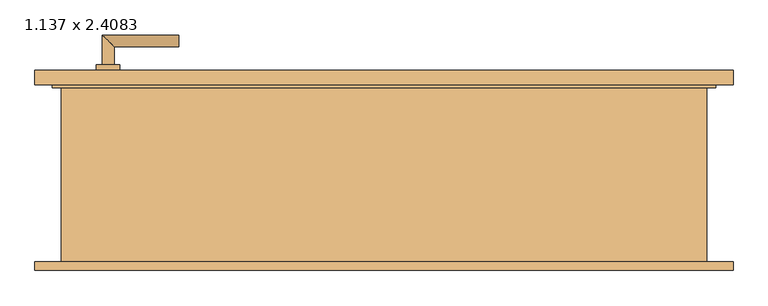
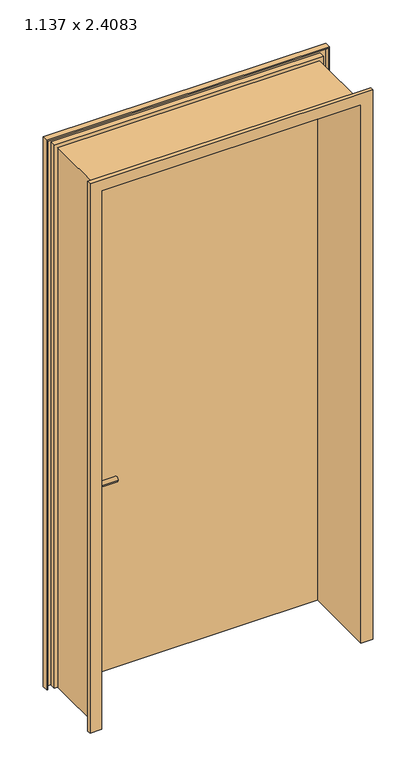
"""IFC4 building model written with IfcOpenShell, lengths in millimetres: door geometry, Drehflügel 1-flg - Stahlzarge : 1.137 x 2.4083."""

import ifcopenshell
import ifcopenshell.guid

model = None  # the IFC model being written
_history = None  # IfcOwnerHistory: only IFC2X3 demands one
_inside = {}  # id of a spatial element -> (the spatial element, [elements in it])
_under = {}  # id of a project, library or spatial element -> (it, [spatial elements below it])
_declared = {}  # id of a project -> (the project, [libraries it declares])
_typed = {}  # id of a type object -> (the type object, [elements of that type])
_made_of = {}  # id of a material, layer set ... -> (it, [elements and type objects made of it])


def new_model(schema):
    """Start an empty IFC model of exactly this schema.

    Asked for "IFC4X3", IfcOpenShell would pick the latest addendum, in which some entities
    have other attributes; the version numbers below select the first issue.
    IFC2X3 requires an IfcOwnerHistory on every rooted entity: one is made here for all.
    """
    global model, _history
    if schema == "IFC4X3":
        model = ifcopenshell.file(schema_version=(4, 3, 0, 0))
    else:
        model = ifcopenshell.file(schema=schema)
    _inside.clear()
    _under.clear()
    _declared.clear()
    _typed.clear()
    _made_of.clear()
    _history = None
    if model.schema == "IFC2X3":
        org = make("IfcOrganization", Name="unknown")
        user = make(
            "IfcPersonAndOrganization",
            ThePerson=make("IfcPerson", FamilyName="unknown"),
            TheOrganization=org,
        )
        app = make(
            "IfcApplication",
            ApplicationDeveloper=org,
            Version="unknown",
            ApplicationFullName="unknown",
            ApplicationIdentifier="unknown",
        )
        _history = make(
            "IfcOwnerHistory",
            OwningUser=user,
            OwningApplication=app,
            ChangeAction="ADDED",
            CreationDate=0,
        )
    return model


def make(cls, **values):
    """One entity of the class cls with the attributes given. An attribute that is None is left unset."""
    return model.create_entity(
        cls, **{name: value for name, value in values.items() if value is not None}
    )


def rooted(cls, **values):
    """An entity with a GlobalId (a new one), such as an element, a storey or a relation."""
    return make(cls, GlobalId=ifcopenshell.guid.new(), OwnerHistory=_history, **values)


def si_unit(unit_type, name, prefix=None):
    """IfcSIUnit, for example si_unit("LENGTHUNIT", "METRE", prefix="MILLI")."""
    return make("IfcSIUnit", UnitType=unit_type, Prefix=prefix, Name=name)


def assignment(units):
    """IfcUnitAssignment: the units of a project."""
    return None if units is None else make("IfcUnitAssignment", Units=units)


def point(xyz):
    """IfcCartesianPoint."""
    return None if xyz is None else make("IfcCartesianPoint", Coordinates=xyz)


def direction(xyz):
    """IfcDirection."""
    return None if xyz is None else make("IfcDirection", DirectionRatios=xyz)


def frame(location, z_axis=None, x_axis=None):
    """IfcAxis2Placement3D, a coordinate frame: its origin and axes. An axis left out is left unset."""
    return make(
        "IfcAxis2Placement3D",
        Location=point(location),
        Axis=direction(z_axis),
        RefDirection=direction(x_axis),
    )


def frame_2d(location, x_axis=None):
    """IfcAxis2Placement2D, a coordinate frame in the plane: its origin and x axis."""
    return make(
        "IfcAxis2Placement2D", Location=point(location), RefDirection=direction(x_axis)
    )


def origin():
    """The frame at (0, 0, 0) with its axes left unset."""
    return frame((0.0, 0.0, 0.0))


def place(relative_to, where):
    """IfcLocalPlacement: puts the frame where relative to a parent placement (None: the world)."""
    return make(
        "IfcLocalPlacement", PlacementRelTo=relative_to, RelativePlacement=where
    )


def context(
    kind, dimensions, precision=None, world=None, true_north=None, identifier=None
):
    """IfcGeometricRepresentationContext, for example the 3D "Model" context."""
    return make(
        "IfcGeometricRepresentationContext",
        ContextIdentifier=identifier,
        ContextType=kind,
        CoordinateSpaceDimension=dimensions,
        Precision=precision,
        WorldCoordinateSystem=world,
        TrueNorth=true_north,
    )


def project(units=None, contexts=None):
    """IfcProject with its units and contexts."""
    return rooted(
        "IfcProject",
        Name="project",
        RepresentationContexts=contexts,
        UnitsInContext=assignment(units),
    )


def spatial(cls, under=None, at=None, **own):
    """A site, building, storey or space (cls), placed at a placement, below another one or the project."""
    s = rooted(cls, ObjectPlacement=at, **own)
    if under is not None:
        _under.setdefault(under.id(), (under, []))[1].append(s)
    return s


def polyline(points):
    """IfcPolyline through the points."""
    return make("IfcPolyline", Points=[point(p) for p in points])


def circle_curve(where, radius):
    """IfcCircle in the frame where."""
    return make("IfcCircle", Position=where, Radius=radius)


def ellipse_curve(where, semi_axis1, semi_axis2):
    """IfcEllipse in the frame where."""
    return make(
        "IfcEllipse", Position=where, SemiAxis1=semi_axis1, SemiAxis2=semi_axis2
    )


def trimmed(basis, trim1, trim2, sense, master):
    """IfcTrimmedCurve: the piece of a basis curve between two trims."""
    return make(
        "IfcTrimmedCurve",
        BasisCurve=basis,
        Trim1=trim1,
        Trim2=trim2,
        SenseAgreement=sense,
        MasterRepresentation=master,
    )


def segment(curve, same_sense, transition):
    """IfcCompositeCurveSegment."""
    return make(
        "IfcCompositeCurveSegment",
        Transition=transition,
        SameSense=same_sense,
        ParentCurve=curve,
    )


def composite_curve(segments, self_intersect=None):
    """IfcCompositeCurve: segments joined end to end."""
    return make("IfcCompositeCurve", Segments=segments, SelfIntersect=self_intersect)


def outline(outer, holes=None, kind="AREA"):
    """IfcArbitraryClosedProfileDef: a profile drawn as a closed curve; with holes, ...WithVoids."""
    if holes is None:
        return make("IfcArbitraryClosedProfileDef", ProfileType=kind, OuterCurve=outer)
    return make(
        "IfcArbitraryProfileDefWithVoids",
        ProfileType=kind,
        OuterCurve=outer,
        InnerCurves=holes,
    )


def extrude(swept, where, along, depth):
    """IfcExtrudedAreaSolid: the profile swept, set in the frame where, extruded along a direction by depth."""
    return make(
        "IfcExtrudedAreaSolid",
        SweptArea=swept,
        Position=where,
        ExtrudedDirection=direction(along),
        Depth=depth,
    )


def faces_of(points, faces, orient=None, outer=None):
    """IfcFace entities. A face is a list of loops; a loop is a list of indices into points, from 0.

    orient and outer hold one flag for each loop. By default every Orientation is true, the
    first loop of a face is its IfcFaceOuterBound and the others are IfcFaceBound.
    """
    made = []
    for i, loops in enumerate(faces):
        bounds = []
        for j, loop in enumerate(loops):
            is_outer = j == 0 if outer is None else outer[i][j]
            bounds.append(
                make(
                    "IfcFaceOuterBound" if is_outer else "IfcFaceBound",
                    Bound=make("IfcPolyLoop", Polygon=[points[k] for k in loop]),
                    Orientation=True if orient is None else orient[i][j],
                )
            )
        made.append(make("IfcFace", Bounds=bounds))
    return made


def faceted_brep(points, faces, orient=None, outer=None, voids=None):
    """IfcFacetedBrep: a solid bounded by flat faces; with voids (closed shells), ...WithVoids."""
    shared = [point(p) for p in points]
    hull = make("IfcClosedShell", CfsFaces=faces_of(shared, faces, orient, outer))
    if voids is None:
        return make("IfcFacetedBrep", Outer=hull)
    return make(
        "IfcFacetedBrepWithVoids",
        Outer=hull,
        Voids=[
            make(cls, CfsFaces=faces_of(shared, fs, o, b)) for cls, fs, o, b in voids
        ],
    )


def shape(context_of_items, identifier, shape_type, items):
    """IfcShapeRepresentation: the items that make up one representation, for example the "Body"."""
    return make(
        "IfcShapeRepresentation",
        ContextOfItems=context_of_items,
        RepresentationIdentifier=identifier,
        RepresentationType=shape_type,
        Items=items,
    )


def source(mapping_origin, context_of_items, identifier, shape_type, items):
    """IfcRepresentationMap: a shape defined once, which mapped items show again and again."""
    return make(
        "IfcRepresentationMap",
        MappingOrigin=mapping_origin,
        MappedRepresentation=shape(context_of_items, identifier, shape_type, items),
    )


def transform(
    local_origin,
    x_axis=None,
    y_axis=None,
    z_axis=None,
    scale=None,
    scale2=None,
    scale3=None,
    uniform=True,
):
    """IfcCartesianTransformationOperator3D, or its non-uniform kind. x_axis, y_axis, z_axis: its Axis1, 2, 3."""
    if uniform:
        return make(
            "IfcCartesianTransformationOperator3D",
            Axis1=direction(x_axis),
            Axis2=direction(y_axis),
            LocalOrigin=point(local_origin),
            Scale=scale,
            Axis3=direction(z_axis),
        )
    return make(
        "IfcCartesianTransformationOperator3DnonUniform",
        Axis1=direction(x_axis),
        Axis2=direction(y_axis),
        LocalOrigin=point(local_origin),
        Scale=scale,
        Axis3=direction(z_axis),
        Scale2=scale2,
        Scale3=scale3,
    )


def mapped(mapping_source, mapping_target):
    """IfcMappedItem: shows the shape of a source again, moved by a transform."""
    return make(
        "IfcMappedItem", MappingSource=mapping_source, MappingTarget=mapping_target
    )


def made_of(thing, what):
    """Note that an element or type object is made of a material, layer set ...; save() writes the relation."""
    if what is not None:
        _made_of.setdefault(what.id(), (what, []))[1].append(thing)
    return thing


def element(
    cls,
    number,
    at=None,
    inside=None,
    cuts=None,
    type_object=None,
    material=None,
    context=None,
    identifier="Body",
    shape_type=None,
    held_by="IfcProductDefinitionShape",
    body=None,
    shapes=None,
    **own,
):
    """One element of the class cls, such as IfcWall. Its Tag is "e" and its number.

    at: its placement. inside: the storey or other place that contains it. cuts: it is an
    opening in that element (IfcRelVoidsElement). A single representation is given by context,
    identifier, shape_type and body (its items); several are given by shapes. held_by: the class
    of the entity that holds the representations. save() writes the other relations.
    """
    e = rooted(cls, Tag="e%d" % number, ObjectPlacement=at, **own)
    if body is not None:
        shapes = [shape(context, identifier, shape_type, body)]
    if shapes is not None:
        e.Representation = make(held_by, Representations=shapes)
    if inside is not None:
        _inside.setdefault(inside.id(), (inside, []))[1].append(e)
    if cuts is not None:
        rooted(
            "IfcRelVoidsElement", RelatingBuildingElement=cuts, RelatedOpeningElement=e
        )
    if type_object is not None:
        _typed.setdefault(type_object.id(), (type_object, []))[1].append(e)
    return made_of(e, material)


def aggregate(whole, parts):
    """IfcRelAggregates: a whole, such as a stair, and the parts it consists of."""
    return rooted("IfcRelAggregates", RelatingObject=whole, RelatedObjects=parts)


def save(model, path):
    """Write the relations noted so far, then the file.

    IfcRelAggregates (storeys below a building ...), IfcRelContainedInSpatialStructure (elements
    in a storey), IfcRelDefinesByType, IfcRelAssociatesMaterial and IfcRelDeclares: one each for
    every whole, place, type object, material and project.
    """
    for whole, parts in _under.values():
        aggregate(whole, parts)
    for where, things in _inside.values():
        rooted(
            "IfcRelContainedInSpatialStructure",
            RelatedElements=things,
            RelatingStructure=where,
        )
    for kind, things in _typed.values():
        rooted("IfcRelDefinesByType", RelatedObjects=things, RelatingType=kind)
    for what, things in _made_of.values():
        rooted("IfcRelAssociatesMaterial", RelatedObjects=things, RelatingMaterial=what)
    for by, libraries in _declared.values():
        rooted("IfcRelDeclares", RelatingContext=by, RelatedDefinitions=libraries)
    model.write(path)


def plane_surface(at):
    """IfcPlane: the flat surface through the origin of the frame at, square to its z axis."""
    return make("IfcPlane", Position=at)


def cylinder_surface(at, radius):
    """IfcCylindricalSurface: all points at the distance radius from the z axis of the frame at."""
    return make("IfcCylindricalSurface", Position=at, Radius=radius)


def advanced_brep(points, edges, surfaces, faces):
    """IfcAdvancedBrep: a solid bounded by faces that lie on surfaces and meet in shared edges.

    An edge is (start, end): straight between two places in points (the first is 0);
    or (start, end, curve); or (start, end, curve, False) where it runs against its curve.
    A face is (place in surfaces, loops), or (place, loops, False) where it looks against
    its surface's normal. A loop lists edges by number (the first is 1), with a minus sign
    where the edge is run from its end to its start. The first loop is the outer one.
    """
    corners = [point(p) for p in points]
    vertices = [make("IfcVertexPoint", VertexGeometry=c) for c in corners]
    made = []
    for start, end, *more in edges:
        made.append(
            make(
                "IfcEdgeCurve",
                EdgeStart=vertices[start],
                EdgeEnd=vertices[end],
                EdgeGeometry=more[0] if more else make("IfcPolyline", Points=[corners[start], corners[end]]),
                SameSense=more[1] if len(more) > 1 else True,
            )
        )
    hull = []
    for where, loops, *sense in faces:
        bounds = []
        for j, loop in enumerate(loops):
            ring = [make("IfcOrientedEdge", EdgeElement=made[abs(k) - 1], Orientation=k > 0) for k in loop]
            bounds.append(
                make(
                    "IfcFaceOuterBound" if j == 0 else "IfcFaceBound",
                    Bound=make("IfcEdgeLoop", EdgeList=ring),
                    Orientation=True,
                )
            )
        hull.append(make("IfcAdvancedFace", Bounds=bounds, FaceSurface=surfaces[where], SameSense=sense[0] if sense else True))
    return make("IfcAdvancedBrep", Outer=make("IfcClosedShell", CfsFaces=hull))


def door_1_137_x_2_4083_873f2a3c(model_context):
    return source(origin(), model_context, "Body", "SolidModel", [
        advanced_brep(
        [(-478.5, 139.4346141, 915.0), (-458.5, 139.4346141, 915.0), (-478.5, 69.4346141, 915.0), (-458.5, 89.4346141, 915.0), (-348.5, 69.4346141, 915.0), (-348.5, 89.4346141, 915.0)],
        [
            (0, 1, circle_curve(frame((-468.5, 139.4346141, 915.0), z_axis=(0.0, 1.0, 0.0), x_axis=(1.0, 0.0, 0.0)), 10.0)),
            (1, 0, circle_curve(frame((-468.5, 139.4346141, 915.0), z_axis=(0.0, 1.0, 0.0), x_axis=(1.0, 0.0, 0.0)), 10.0)),
            (0, 2),
            (2, 3, ellipse_curve(frame((-468.5, 79.4346141, 915.0), z_axis=(-0.7071067811865385, 0.7071067811865565, 0.0), x_axis=(0.7071067811865563, 0.7071067811865386, 0.0)), 14.1421356, 10.0)),
            (3, 1),
            (3, 2, ellipse_curve(frame((-468.5, 79.4346141, 915.0), z_axis=(-0.7071067811865385, 0.7071067811865565, 0.0), x_axis=(0.7071067811865563, 0.7071067811865386, 0.0)), 14.1421356, 10.0)),
            (4, 5, circle_curve(frame((-348.5, 79.4346141, 915.0), z_axis=(1.0, 0.0, 0.0), x_axis=(0.0, 1.0, 0.0)), 10.0)),
            (5, 4, circle_curve(frame((-348.5, 79.4346141, 915.0), z_axis=(1.0, 0.0, 0.0), x_axis=(0.0, 1.0, 0.0)), 10.0)),
            (2, 4),
            (5, 3),
        ],
        [
            plane_surface(frame((-468.5, 139.4346141, -372.7526403), z_axis=(0.0, 1.0, 0.0), x_axis=(0.0, 0.0, 1.0))),
            cylinder_surface(frame((-468.5, 139.4346141, 915.0), z_axis=(0.0, 1.0, 0.0), x_axis=(1.0, 0.0, 0.0)), 10.0),
            plane_surface(frame((-348.5, 79.4346141, -372.7526403), z_axis=(1.0, 0.0, 0.0), x_axis=(0.0, 0.0, 1.0))),
            cylinder_surface(frame((-468.5, 79.4346141, 915.0), z_axis=(-1.0, 0.0, 0.0), x_axis=(0.0, 1.0, 0.0)), 10.0),
        ],
        [
            (0, [[1, 2]]),
            (1, [[-1, 3, 4, 5]]),
            (1, [[-2, -5, 6, -3]]),
            (2, [[7, 8]]),
            (3, [[-4, 9, -8, 10]]),
            (3, [[-6, -10, -7, -9]]),
        ],
    ),
        advanced_brep(
        [(-458.5, 199.4346141, 915.0), (-478.5, 199.4346141, 915.0), (-458.5, 229.4346141, 915.0), (-478.5, 249.4346141, 915.0), (-348.5, 229.4346141, 915.0), (-348.5, 249.4346141, 915.0)],
        [
            (0, 1, circle_curve(frame((-468.5, 199.4346141, 915.0), z_axis=(0.0, -1.0, 0.0), x_axis=(-1.0, 0.0, 0.0)), 10.0)),
            (1, 0, circle_curve(frame((-468.5, 199.4346141, 915.0), z_axis=(0.0, -1.0, 0.0), x_axis=(-1.0, 0.0, 0.0)), 10.0)),
            (0, 2),
            (2, 3, ellipse_curve(frame((-468.5, 239.4346141, 915.0), z_axis=(-0.7071067811865475, -0.7071067811865475, 0.0), x_axis=(0.7071067811865474, -0.7071067811865476, 0.0)), 14.1421356, 10.0)),
            (3, 1),
            (3, 2, ellipse_curve(frame((-468.5, 239.4346141, 915.0), z_axis=(-0.7071067811865475, -0.7071067811865475, 0.0), x_axis=(0.7071067811865474, -0.7071067811865476, 0.0)), 14.1421356, 10.0)),
            (4, 5, circle_curve(frame((-348.5, 239.4346141, 915.0), z_axis=(1.0, 0.0, 0.0), x_axis=(0.0, 1.0, 0.0)), 10.0)),
            (5, 4, circle_curve(frame((-348.5, 239.4346141, 915.0), z_axis=(1.0, 0.0, 0.0), x_axis=(0.0, 1.0, 0.0)), 10.0)),
            (2, 4),
            (5, 3),
        ],
        [
            plane_surface(frame((-468.5, 199.4346141, -372.7526403), z_axis=(0.0, -1.0, 0.0), x_axis=(0.0, 0.0, 1.0))),
            cylinder_surface(frame((-468.5, 199.4346141, 915.0), z_axis=(0.0, -1.0, 0.0), x_axis=(-1.0, 0.0, 0.0)), 10.0),
            plane_surface(frame((-348.5, 239.4346141, -372.7526403), z_axis=(1.0, 0.0, 0.0), x_axis=(0.0, 0.0, 1.0))),
            cylinder_surface(frame((-468.5, 239.4346141, 915.0), z_axis=(-1.0, 0.0, 0.0), x_axis=(0.0, 1.0, 0.0)), 10.0),
        ],
        [
            (0, [[1, 2]]),
            (1, [[-1, 3, 4, 5]]),
            (1, [[-2, -5, 6, -3]]),
            (2, [[7, 8]]),
            (3, [[-4, 9, -8, 10]]),
            (3, [[-6, -10, -7, -9]]),
        ],
    ),
        extrude(outline(composite_curve([segment(trimmed(circle_curve(frame_2d((915.0, -468.5)), 20.0), [point((915.0, -488.5))], [point((915.0, -448.5))], False, "CARTESIAN"), True, "CONTINUOUS"), segment(trimmed(circle_curve(frame_2d((915.0, -468.5)), 20.0), [point((915.0, -448.5))], [point((915.0, -488.5))], False, "CARTESIAN"), True, "CONTINUOUS")], self_intersect=False)), frame((0.0, 129.4346141, 0.0), z_axis=(0.0, 1.0, 0.0), x_axis=(0.0, 0.0, 1.0)), (0.0, 0.0, 1.0), 10.0),
        extrude(outline(composite_curve([segment(trimmed(circle_curve(frame_2d((915.0, -468.5)), 20.0), [point((915.0, -488.5))], [point((915.0, -448.5))], False, "CARTESIAN"), True, "CONTINUOUS"), segment(trimmed(circle_curve(frame_2d((915.0, -468.5)), 20.0), [point((915.0, -448.5))], [point((915.0, -488.5))], False, "CARTESIAN"), True, "CONTINUOUS")], self_intersect=False)), frame((0.0, 189.4346141, 0.0), z_axis=(0.0, 1.0, 0.0), x_axis=(0.0, 0.0, 1.0)), (0.0, 0.0, 1.0), 10.0),
        extrude(outline(polyline([(558.5, 164.4346141), (-558.5, 164.4346141), (-558.5, 189.4346141), (558.5, 189.4346141), (558.5, 164.4346141)])), frame((0.0, 0.0, 15.0), z_axis=(0.0, 0.0, 1.0), x_axis=(1.0, 0.0, 0.0)), (0.0, 0.0, 1.0), 2398.3),
        faceted_brep([(592.9603207, -150.5653859, 15.0), (543.5, -150.5653859, 15.0), (543.5, 164.4346141, 15.0), (558.5, 164.4346141, 15.0), (558.5, 189.4346141, 15.0), (592.9603207, 189.4346141, 15.0), (592.9603207, 164.4346141, 15.0), (587.9603207, 164.4346141, 15.0), (587.9603207, 184.4346141, 15.0), (563.5, 184.4346141, 15.0), (563.5, 159.4346141, 15.0), (548.5, 159.4346141, 15.0), (548.5, -145.5653859, 15.0), (587.9603207, -145.5653859, 15.0), (587.9603207, -135.5653859, 15.0), (592.9603207, -135.5653859, 15.0), (592.9603207, -150.5653859, 2447.7603207), (-592.9603207, -150.5653859, 2447.7603207), (-592.9603207, -150.5653859, 15.0), (-543.5, -150.5653859, 15.0), (-543.5, -150.5653859, 2398.3), (543.5, -150.5653859, 2398.3), (543.5, 164.4346141, 2398.3), (-543.5, 164.4346141, 2398.3), (-543.5, 164.4346141, 15.0), (-558.5, 164.4346141, 15.0), (-558.5, 164.4346141, 2413.3), (558.5, 164.4346141, 2413.3), (558.5, 189.4346141, 2413.3), (-558.5, 189.4346141, 2413.3), (-558.5, 189.4346141, 15.0), (-592.9603207, 189.4346141, 15.0), (-592.9603207, 189.4346141, 2447.7603207), (592.9603207, 189.4346141, 2447.7603207), (592.9603207, 164.4346141, 2447.7603207), (-592.9603207, 164.4346141, 2447.7603207), (-592.9603207, 164.4346141, 15.0), (-587.9603207, 164.4346141, 15.0), (-587.9603207, 164.4346141, 2442.7603207), (587.9603207, 164.4346141, 2442.7603207), (587.9603207, 184.4346141, 2442.7603207), (-587.9603207, 184.4346141, 2442.7603207), (-587.9603207, 184.4346141, 15.0), (-563.5, 184.4346141, 15.0), (-563.5, 184.4346141, 2418.3), (563.5, 184.4346141, 2418.3), (563.5, 159.4346141, 2418.3), (-563.5, 159.4346141, 2418.3), (-563.5, 159.4346141, 15.0), (-548.5, 159.4346141, 15.0), (-548.5, 159.4346141, 2403.3), (548.5, 159.4346141, 2403.3), (548.5, -145.5653859, 2403.3), (-548.5, -145.5653859, 2403.3), (-548.5, -145.5653859, 15.0), (-587.9603207, -145.5653859, 15.0), (-587.9603207, -145.5653859, 2442.7603207), (587.9603207, -145.5653859, 2442.7603207), (587.9603207, -135.5653859, 2442.7603207), (-587.9603207, -135.5653859, 2442.7603207), (-587.9603207, -135.5653859, 15.0), (-592.9603207, -135.5653859, 15.0), (-592.9603207, -135.5653859, 2447.7603207), (592.9603207, -135.5653859, 2447.7603207)], [[[0, 1, 2, 3, 4, 5, 6, 7, 8, 9, 10, 11, 12, 13, 14, 15]], [[1, 0, 16, 17, 18, 19, 20, 21]], [[2, 1, 21, 22]], [[3, 2, 22, 23, 24, 25, 26, 27]], [[4, 3, 27, 28]], [[5, 4, 28, 29, 30, 31, 32, 33]], [[6, 5, 33, 34]], [[7, 6, 34, 35, 36, 37, 38, 39]], [[8, 7, 39, 40]], [[9, 8, 40, 41, 42, 43, 44, 45]], [[10, 9, 45, 46]], [[11, 10, 46, 47, 48, 49, 50, 51]], [[12, 11, 51, 52]], [[13, 12, 52, 53, 54, 55, 56, 57]], [[14, 13, 57, 58]], [[15, 14, 58, 59, 60, 61, 62, 63]], [[0, 15, 63, 16]], [[17, 62, 61, 18]], [[18, 61, 60, 55, 54, 49, 48, 43, 42, 37, 36, 31, 30, 25, 24, 19]], [[23, 20, 19, 24]], [[29, 26, 25, 30]], [[35, 32, 31, 36]], [[41, 38, 37, 42]], [[47, 44, 43, 48]], [[53, 50, 49, 54]], [[59, 56, 55, 60]], [[22, 21, 20, 23]], [[28, 27, 26, 29]], [[34, 33, 32, 35]], [[40, 39, 38, 41]], [[46, 45, 44, 47]], [[52, 51, 50, 53]], [[58, 57, 56, 59]], [[16, 63, 62, 17]]]),
    ])


if __name__ == "__main__":
    model = new_model("IFC4")
    model_context = context("Model", 3, world=origin())
    ifc_project = project(units=[si_unit("LENGTHUNIT", "METRE", prefix="MILLI")], contexts=[model_context])
    site = spatial("IfcSite", under=ifc_project)
    building = spatial("IfcBuilding", under=site)
    placement = place(None, origin())
    door_1_137_x_2_4083_shape = door_1_137_x_2_4083_873f2a3c(model_context)
    element("IfcDoor", 1, ObjectType="Drehflügel 1-flg - Stahlzarge : 1.137 x 2.4083", at=placement, inside=building, context=model_context, shape_type="MappedRepresentation", body=[
        mapped(door_1_137_x_2_4083_shape, transform((0.0, 0.0, 0.0), x_axis=(1.0, 0.0, 0.0), y_axis=(0.0, 1.0, 0.0), z_axis=(0.0, 0.0, 1.0))),
    ])
    save(model, "model.ifc")

# Revit data of these elements
# Type "Drehflügel 1-flg - Stahlzarge : 1.137 x 2.4083"
#   Type Mark = "21"
#   Operation = "SingleSwingRight"
#   Keynote = "16.03"
#   Analytic Construction = "Metall"
#   Thermal Resistance (R) = 0.270117 (m²·K)/W
#   Heat Transfer Coefficient (U) = 3.7021 W/(m²·K)
#   Rough Width = 1.137 m
#   Rough Height [instance default] = 2.5083 m
#   Höhe Türgriff [instance default] = 0.900 m
#   Height = 2.4083 m
#   Fußbodenaufbau [instance default] = 0.100 m
#   Width = 1.137 m
#   Sichtbarkeit Sturzlinien [instance default] = yes
#   Türgriff auswählen [instance default] = element 221079
#   Türgriff [instance default] = none
#   Türflügel [instance default] = none
#   Rahmen/Pfosten [instance default] = Metall - Lackiert - Grau
#   Visual Light Transmittance = 0
#   Solar Heat Gain Coefficient = 0
#   Function = (empty or 0)
#   Wall Closure = (empty or 0)
# Element 1 (IfcDoor, "Drehflügel 1-flg - Stahlzarge : 1.137 x 2.4083")
#   Rough Height = 2.4233 m
#   Fußbodenaufbau = 0.015 m
#   Materials on its faces: "Metall - Lackiert - Grau", "Metall - Chrom", "Holz - Birke"
# Materials
#   "Metall - Lackiert - Grau": class "Farbe 1", colour RGB 98 98 98, transparency 0, Cost = 0
#   "Metall - Chrom": class "Metall", colour RGB 247 247 247, transparency 0, Cost = 0
#   "Holz - Birke": class "Holz", colour RGB 213 164 103, transparency 0, Cost = 0
